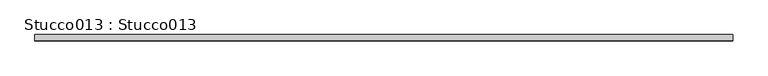
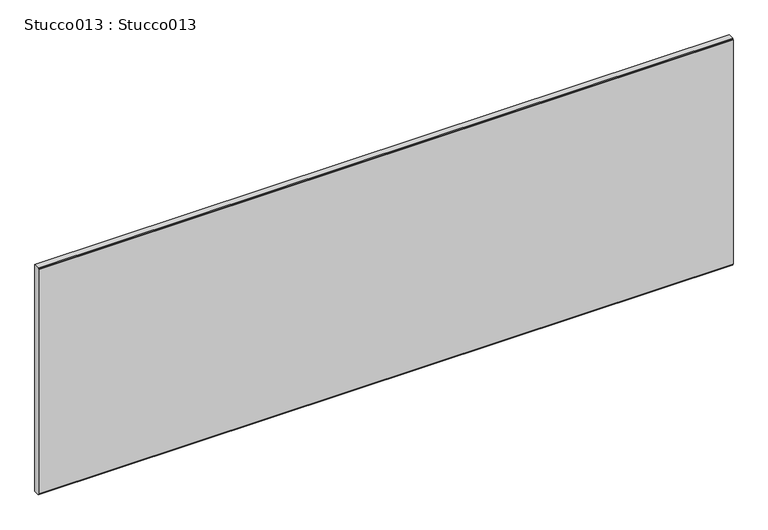
"""IFC4 building model written with IfcOpenShell, lengths in millimetres: proxy geometry, Stucco013 : Stucco013."""

import ifcopenshell
import ifcopenshell.guid

model = None  # the IFC model being written
_history = None  # IfcOwnerHistory: only IFC2X3 demands one
_inside = {}  # id of a spatial element -> (the spatial element, [elements in it])
_under = {}  # id of a project, library or spatial element -> (it, [spatial elements below it])
_declared = {}  # id of a project -> (the project, [libraries it declares])
_typed = {}  # id of a type object -> (the type object, [elements of that type])
_made_of = {}  # id of a material, layer set ... -> (it, [elements and type objects made of it])


def new_model(schema):
    """Start an empty IFC model of exactly this schema.

    Asked for "IFC4X3", IfcOpenShell would pick the latest addendum, in which some entities
    have other attributes; the version numbers below select the first issue.
    IFC2X3 requires an IfcOwnerHistory on every rooted entity: one is made here for all.
    """
    global model, _history
    if schema == "IFC4X3":
        model = ifcopenshell.file(schema_version=(4, 3, 0, 0))
    else:
        model = ifcopenshell.file(schema=schema)
    _inside.clear()
    _under.clear()
    _declared.clear()
    _typed.clear()
    _made_of.clear()
    _history = None
    if model.schema == "IFC2X3":
        org = make("IfcOrganization", Name="unknown")
        user = make(
            "IfcPersonAndOrganization",
            ThePerson=make("IfcPerson", FamilyName="unknown"),
            TheOrganization=org,
        )
        app = make(
            "IfcApplication",
            ApplicationDeveloper=org,
            Version="unknown",
            ApplicationFullName="unknown",
            ApplicationIdentifier="unknown",
        )
        _history = make(
            "IfcOwnerHistory",
            OwningUser=user,
            OwningApplication=app,
            ChangeAction="ADDED",
            CreationDate=0,
        )
    return model


def make(cls, **values):
    """One entity of the class cls with the attributes given. An attribute that is None is left unset."""
    return model.create_entity(
        cls, **{name: value for name, value in values.items() if value is not None}
    )


def rooted(cls, **values):
    """An entity with a GlobalId (a new one), such as an element, a storey or a relation."""
    return make(cls, GlobalId=ifcopenshell.guid.new(), OwnerHistory=_history, **values)


def si_unit(unit_type, name, prefix=None):
    """IfcSIUnit, for example si_unit("LENGTHUNIT", "METRE", prefix="MILLI")."""
    return make("IfcSIUnit", UnitType=unit_type, Prefix=prefix, Name=name)


def assignment(units):
    """IfcUnitAssignment: the units of a project."""
    return None if units is None else make("IfcUnitAssignment", Units=units)


def point(xyz):
    """IfcCartesianPoint."""
    return None if xyz is None else make("IfcCartesianPoint", Coordinates=xyz)


def direction(xyz):
    """IfcDirection."""
    return None if xyz is None else make("IfcDirection", DirectionRatios=xyz)


def frame(location, z_axis=None, x_axis=None):
    """IfcAxis2Placement3D, a coordinate frame: its origin and axes. An axis left out is left unset."""
    return make(
        "IfcAxis2Placement3D",
        Location=point(location),
        Axis=direction(z_axis),
        RefDirection=direction(x_axis),
    )


def origin():
    """The frame at (0, 0, 0) with its axes left unset."""
    return frame((0.0, 0.0, 0.0))


def place(relative_to, where):
    """IfcLocalPlacement: puts the frame where relative to a parent placement (None: the world)."""
    return make(
        "IfcLocalPlacement", PlacementRelTo=relative_to, RelativePlacement=where
    )


def context(
    kind, dimensions, precision=None, world=None, true_north=None, identifier=None
):
    """IfcGeometricRepresentationContext, for example the 3D "Model" context."""
    return make(
        "IfcGeometricRepresentationContext",
        ContextIdentifier=identifier,
        ContextType=kind,
        CoordinateSpaceDimension=dimensions,
        Precision=precision,
        WorldCoordinateSystem=world,
        TrueNorth=true_north,
    )


def project(units=None, contexts=None):
    """IfcProject with its units and contexts."""
    return rooted(
        "IfcProject",
        Name="project",
        RepresentationContexts=contexts,
        UnitsInContext=assignment(units),
    )


def spatial(cls, under=None, at=None, **own):
    """A site, building, storey or space (cls), placed at a placement, below another one or the project."""
    s = rooted(cls, ObjectPlacement=at, **own)
    if under is not None:
        _under.setdefault(under.id(), (under, []))[1].append(s)
    return s


def polyline(points):
    """IfcPolyline through the points."""
    return make("IfcPolyline", Points=[point(p) for p in points])


def outline(outer, holes=None, kind="AREA"):
    """IfcArbitraryClosedProfileDef: a profile drawn as a closed curve; with holes, ...WithVoids."""
    if holes is None:
        return make("IfcArbitraryClosedProfileDef", ProfileType=kind, OuterCurve=outer)
    return make(
        "IfcArbitraryProfileDefWithVoids",
        ProfileType=kind,
        OuterCurve=outer,
        InnerCurves=holes,
    )


def extrude(swept, where, along, depth):
    """IfcExtrudedAreaSolid: the profile swept, set in the frame where, extruded along a direction by depth."""
    return make(
        "IfcExtrudedAreaSolid",
        SweptArea=swept,
        Position=where,
        ExtrudedDirection=direction(along),
        Depth=depth,
    )


def shape(context_of_items, identifier, shape_type, items):
    """IfcShapeRepresentation: the items that make up one representation, for example the "Body"."""
    return make(
        "IfcShapeRepresentation",
        ContextOfItems=context_of_items,
        RepresentationIdentifier=identifier,
        RepresentationType=shape_type,
        Items=items,
    )


def source(mapping_origin, context_of_items, identifier, shape_type, items):
    """IfcRepresentationMap: a shape defined once, which mapped items show again and again."""
    return make(
        "IfcRepresentationMap",
        MappingOrigin=mapping_origin,
        MappedRepresentation=shape(context_of_items, identifier, shape_type, items),
    )


def transform(
    local_origin,
    x_axis=None,
    y_axis=None,
    z_axis=None,
    scale=None,
    scale2=None,
    scale3=None,
    uniform=True,
):
    """IfcCartesianTransformationOperator3D, or its non-uniform kind. x_axis, y_axis, z_axis: its Axis1, 2, 3."""
    if uniform:
        return make(
            "IfcCartesianTransformationOperator3D",
            Axis1=direction(x_axis),
            Axis2=direction(y_axis),
            LocalOrigin=point(local_origin),
            Scale=scale,
            Axis3=direction(z_axis),
        )
    return make(
        "IfcCartesianTransformationOperator3DnonUniform",
        Axis1=direction(x_axis),
        Axis2=direction(y_axis),
        LocalOrigin=point(local_origin),
        Scale=scale,
        Axis3=direction(z_axis),
        Scale2=scale2,
        Scale3=scale3,
    )


def mapped(mapping_source, mapping_target):
    """IfcMappedItem: shows the shape of a source again, moved by a transform."""
    return make(
        "IfcMappedItem", MappingSource=mapping_source, MappingTarget=mapping_target
    )


def made_of(thing, what):
    """Note that an element or type object is made of a material, layer set ...; save() writes the relation."""
    if what is not None:
        _made_of.setdefault(what.id(), (what, []))[1].append(thing)
    return thing


def element(
    cls,
    number,
    at=None,
    inside=None,
    cuts=None,
    type_object=None,
    material=None,
    context=None,
    identifier="Body",
    shape_type=None,
    held_by="IfcProductDefinitionShape",
    body=None,
    shapes=None,
    **own,
):
    """One element of the class cls, such as IfcWall. Its Tag is "e" and its number.

    at: its placement. inside: the storey or other place that contains it. cuts: it is an
    opening in that element (IfcRelVoidsElement). A single representation is given by context,
    identifier, shape_type and body (its items); several are given by shapes. held_by: the class
    of the entity that holds the representations. save() writes the other relations.
    """
    e = rooted(cls, Tag="e%d" % number, ObjectPlacement=at, **own)
    if body is not None:
        shapes = [shape(context, identifier, shape_type, body)]
    if shapes is not None:
        e.Representation = make(held_by, Representations=shapes)
    if inside is not None:
        _inside.setdefault(inside.id(), (inside, []))[1].append(e)
    if cuts is not None:
        rooted(
            "IfcRelVoidsElement", RelatingBuildingElement=cuts, RelatedOpeningElement=e
        )
    if type_object is not None:
        _typed.setdefault(type_object.id(), (type_object, []))[1].append(e)
    return made_of(e, material)


def aggregate(whole, parts):
    """IfcRelAggregates: a whole, such as a stair, and the parts it consists of."""
    return rooted("IfcRelAggregates", RelatingObject=whole, RelatedObjects=parts)


def save(model, path):
    """Write the relations noted so far, then the file.

    IfcRelAggregates (storeys below a building ...), IfcRelContainedInSpatialStructure (elements
    in a storey), IfcRelDefinesByType, IfcRelAssociatesMaterial and IfcRelDeclares: one each for
    every whole, place, type object, material and project.
    """
    for whole, parts in _under.values():
        aggregate(whole, parts)
    for where, things in _inside.values():
        rooted(
            "IfcRelContainedInSpatialStructure",
            RelatedElements=things,
            RelatingStructure=where,
        )
    for kind, things in _typed.values():
        rooted("IfcRelDefinesByType", RelatedObjects=things, RelatingType=kind)
    for what, things in _made_of.values():
        rooted("IfcRelAssociatesMaterial", RelatedObjects=things, RelatingMaterial=what)
    for by, libraries in _declared.values():
        rooted("IfcRelDeclares", RelatingContext=by, RelatedDefinitions=libraries)
    model.write(path)


def stucco013_stucco013_f6ea3313(model_context):
    return source(origin(), model_context, "Body", "SweptSolid", [
        extrude(outline(polyline([(-4684.6182816, 39037.046675), (-4685.8882816, 39037.046675), (-4685.8882816, 39720.5548875), (-4684.6182816, 39720.5548875), (-4684.6182816, 39724.0346875), (-4667.6543336, 39724.0346875), (-4667.6543336, 39033.566875), (-4684.6182816, 39033.566875), (-4684.6182816, 39037.046675)])), frame((12383.0178845, 0.0, 0.0), z_axis=(1.0, 0.0, 0.0), x_axis=(0.0, 1.0, 0.0)), (0.0, 0.0, 1.0), 2000.0),
    ])


if __name__ == "__main__":
    model = new_model("IFC4")
    model_context = context("Model", 3, world=origin())
    ifc_project = project(units=[si_unit("LENGTHUNIT", "METRE", prefix="MILLI")], contexts=[model_context])
    site = spatial("IfcSite", under=ifc_project)
    building = spatial("IfcBuilding", under=site)
    placement = place(None, origin())
    stucco013_stucco013_shape = stucco013_stucco013_f6ea3313(model_context)
    element("IfcBuildingElementProxy", 1, Name="Stucco013 : Stucco013", ObjectType="Stucco013 : Stucco013", at=placement, inside=building, context=model_context, shape_type="MappedRepresentation", body=[
        mapped(stucco013_stucco013_shape, transform((0.0, 0.0, 0.0), x_axis=(1.0, 0.0, 0.0), y_axis=(0.0, 1.0, 0.0), z_axis=(0.0, 0.0, 1.0))),
    ])
    save(model, "model.ifc")

# Revit data of these elements
# Type "Stucco013 : Stucco013"
#   NameOverride = "Stucco013"
# Element 1 (IfcBuildingElementProxy, "Stucco013 : Stucco013")
#   Materials on its faces: "7/8\" SMOOTH TROWEL EXTERIOR STUCCO"
# Materials
#   "7/8\" SMOOTH TROWEL EXTERIOR STUCCO": class "Unassigned", colour RGB 255 255 255, transparency 0, Cost = 0
